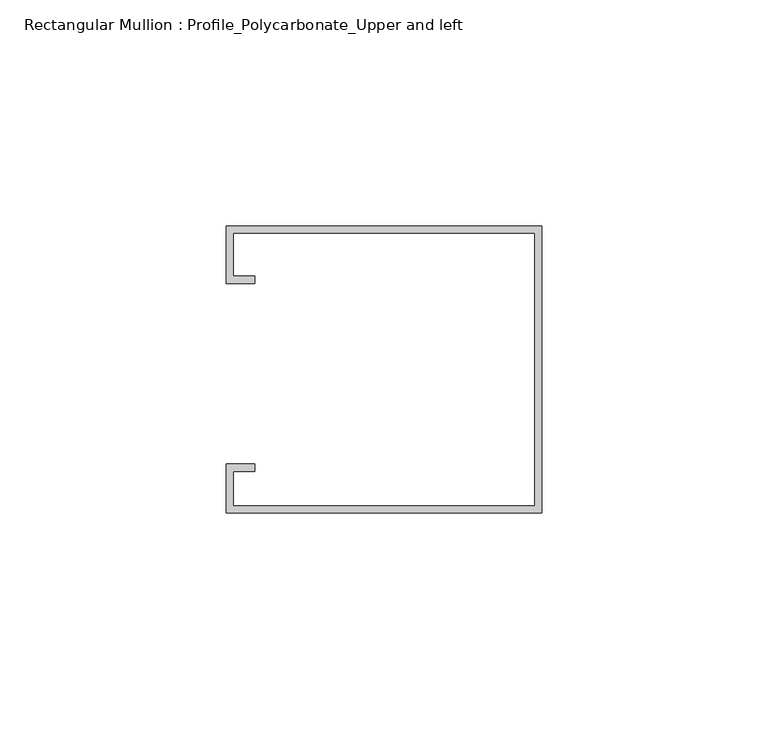
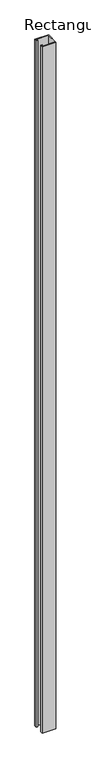
"""IFC4 building model written with IfcOpenShell, lengths in millimetres: member geometry, Rectangular Mullion : Profile_Polycarbonate_Upper and left."""

import ifcopenshell
import ifcopenshell.guid

model = None  # the IFC model being written
_history = None  # IfcOwnerHistory: only IFC2X3 demands one
_inside = {}  # id of a spatial element -> (the spatial element, [elements in it])
_under = {}  # id of a project, library or spatial element -> (it, [spatial elements below it])
_declared = {}  # id of a project -> (the project, [libraries it declares])
_typed = {}  # id of a type object -> (the type object, [elements of that type])
_made_of = {}  # id of a material, layer set ... -> (it, [elements and type objects made of it])


def new_model(schema):
    """Start an empty IFC model of exactly this schema.

    Asked for "IFC4X3", IfcOpenShell would pick the latest addendum, in which some entities
    have other attributes; the version numbers below select the first issue.
    IFC2X3 requires an IfcOwnerHistory on every rooted entity: one is made here for all.
    """
    global model, _history
    if schema == "IFC4X3":
        model = ifcopenshell.file(schema_version=(4, 3, 0, 0))
    else:
        model = ifcopenshell.file(schema=schema)
    _inside.clear()
    _under.clear()
    _declared.clear()
    _typed.clear()
    _made_of.clear()
    _history = None
    if model.schema == "IFC2X3":
        org = make("IfcOrganization", Name="unknown")
        user = make(
            "IfcPersonAndOrganization",
            ThePerson=make("IfcPerson", FamilyName="unknown"),
            TheOrganization=org,
        )
        app = make(
            "IfcApplication",
            ApplicationDeveloper=org,
            Version="unknown",
            ApplicationFullName="unknown",
            ApplicationIdentifier="unknown",
        )
        _history = make(
            "IfcOwnerHistory",
            OwningUser=user,
            OwningApplication=app,
            ChangeAction="ADDED",
            CreationDate=0,
        )
    return model


def make(cls, **values):
    """One entity of the class cls with the attributes given. An attribute that is None is left unset."""
    return model.create_entity(
        cls, **{name: value for name, value in values.items() if value is not None}
    )


def rooted(cls, **values):
    """An entity with a GlobalId (a new one), such as an element, a storey or a relation."""
    return make(cls, GlobalId=ifcopenshell.guid.new(), OwnerHistory=_history, **values)


def si_unit(unit_type, name, prefix=None):
    """IfcSIUnit, for example si_unit("LENGTHUNIT", "METRE", prefix="MILLI")."""
    return make("IfcSIUnit", UnitType=unit_type, Prefix=prefix, Name=name)


def assignment(units):
    """IfcUnitAssignment: the units of a project."""
    return None if units is None else make("IfcUnitAssignment", Units=units)


def point(xyz):
    """IfcCartesianPoint."""
    return None if xyz is None else make("IfcCartesianPoint", Coordinates=xyz)


def direction(xyz):
    """IfcDirection."""
    return None if xyz is None else make("IfcDirection", DirectionRatios=xyz)


def frame(location, z_axis=None, x_axis=None):
    """IfcAxis2Placement3D, a coordinate frame: its origin and axes. An axis left out is left unset."""
    return make(
        "IfcAxis2Placement3D",
        Location=point(location),
        Axis=direction(z_axis),
        RefDirection=direction(x_axis),
    )


def origin():
    """The frame at (0, 0, 0) with its axes left unset."""
    return frame((0.0, 0.0, 0.0))


def place(relative_to, where):
    """IfcLocalPlacement: puts the frame where relative to a parent placement (None: the world)."""
    return make(
        "IfcLocalPlacement", PlacementRelTo=relative_to, RelativePlacement=where
    )


def context(
    kind, dimensions, precision=None, world=None, true_north=None, identifier=None
):
    """IfcGeometricRepresentationContext, for example the 3D "Model" context."""
    return make(
        "IfcGeometricRepresentationContext",
        ContextIdentifier=identifier,
        ContextType=kind,
        CoordinateSpaceDimension=dimensions,
        Precision=precision,
        WorldCoordinateSystem=world,
        TrueNorth=true_north,
    )


def project(units=None, contexts=None):
    """IfcProject with its units and contexts."""
    return rooted(
        "IfcProject",
        Name="project",
        RepresentationContexts=contexts,
        UnitsInContext=assignment(units),
    )


def spatial(cls, under=None, at=None, **own):
    """A site, building, storey or space (cls), placed at a placement, below another one or the project."""
    s = rooted(cls, ObjectPlacement=at, **own)
    if under is not None:
        _under.setdefault(under.id(), (under, []))[1].append(s)
    return s


def polyline(points):
    """IfcPolyline through the points."""
    return make("IfcPolyline", Points=[point(p) for p in points])


def outline(outer, holes=None, kind="AREA"):
    """IfcArbitraryClosedProfileDef: a profile drawn as a closed curve; with holes, ...WithVoids."""
    if holes is None:
        return make("IfcArbitraryClosedProfileDef", ProfileType=kind, OuterCurve=outer)
    return make(
        "IfcArbitraryProfileDefWithVoids",
        ProfileType=kind,
        OuterCurve=outer,
        InnerCurves=holes,
    )


def extrude(swept, where, along, depth):
    """IfcExtrudedAreaSolid: the profile swept, set in the frame where, extruded along a direction by depth."""
    return make(
        "IfcExtrudedAreaSolid",
        SweptArea=swept,
        Position=where,
        ExtrudedDirection=direction(along),
        Depth=depth,
    )


def shape(context_of_items, identifier, shape_type, items):
    """IfcShapeRepresentation: the items that make up one representation, for example the "Body"."""
    return make(
        "IfcShapeRepresentation",
        ContextOfItems=context_of_items,
        RepresentationIdentifier=identifier,
        RepresentationType=shape_type,
        Items=items,
    )


def source(mapping_origin, context_of_items, identifier, shape_type, items):
    """IfcRepresentationMap: a shape defined once, which mapped items show again and again."""
    return make(
        "IfcRepresentationMap",
        MappingOrigin=mapping_origin,
        MappedRepresentation=shape(context_of_items, identifier, shape_type, items),
    )


def transform(
    local_origin,
    x_axis=None,
    y_axis=None,
    z_axis=None,
    scale=None,
    scale2=None,
    scale3=None,
    uniform=True,
):
    """IfcCartesianTransformationOperator3D, or its non-uniform kind. x_axis, y_axis, z_axis: its Axis1, 2, 3."""
    if uniform:
        return make(
            "IfcCartesianTransformationOperator3D",
            Axis1=direction(x_axis),
            Axis2=direction(y_axis),
            LocalOrigin=point(local_origin),
            Scale=scale,
            Axis3=direction(z_axis),
        )
    return make(
        "IfcCartesianTransformationOperator3DnonUniform",
        Axis1=direction(x_axis),
        Axis2=direction(y_axis),
        LocalOrigin=point(local_origin),
        Scale=scale,
        Axis3=direction(z_axis),
        Scale2=scale2,
        Scale3=scale3,
    )


def mapped(mapping_source, mapping_target):
    """IfcMappedItem: shows the shape of a source again, moved by a transform."""
    return make(
        "IfcMappedItem", MappingSource=mapping_source, MappingTarget=mapping_target
    )


def made_of(thing, what):
    """Note that an element or type object is made of a material, layer set ...; save() writes the relation."""
    if what is not None:
        _made_of.setdefault(what.id(), (what, []))[1].append(thing)
    return thing


def element(
    cls,
    number,
    at=None,
    inside=None,
    cuts=None,
    type_object=None,
    material=None,
    context=None,
    identifier="Body",
    shape_type=None,
    held_by="IfcProductDefinitionShape",
    body=None,
    shapes=None,
    **own,
):
    """One element of the class cls, such as IfcWall. Its Tag is "e" and its number.

    at: its placement. inside: the storey or other place that contains it. cuts: it is an
    opening in that element (IfcRelVoidsElement). A single representation is given by context,
    identifier, shape_type and body (its items); several are given by shapes. held_by: the class
    of the entity that holds the representations. save() writes the other relations.
    """
    e = rooted(cls, Tag="e%d" % number, ObjectPlacement=at, **own)
    if body is not None:
        shapes = [shape(context, identifier, shape_type, body)]
    if shapes is not None:
        e.Representation = make(held_by, Representations=shapes)
    if inside is not None:
        _inside.setdefault(inside.id(), (inside, []))[1].append(e)
    if cuts is not None:
        rooted(
            "IfcRelVoidsElement", RelatingBuildingElement=cuts, RelatedOpeningElement=e
        )
    if type_object is not None:
        _typed.setdefault(type_object.id(), (type_object, []))[1].append(e)
    return made_of(e, material)


def aggregate(whole, parts):
    """IfcRelAggregates: a whole, such as a stair, and the parts it consists of."""
    return rooted("IfcRelAggregates", RelatingObject=whole, RelatedObjects=parts)


def save(model, path):
    """Write the relations noted so far, then the file.

    IfcRelAggregates (storeys below a building ...), IfcRelContainedInSpatialStructure (elements
    in a storey), IfcRelDefinesByType, IfcRelAssociatesMaterial and IfcRelDeclares: one each for
    every whole, place, type object, material and project.
    """
    for whole, parts in _under.values():
        aggregate(whole, parts)
    for where, things in _inside.values():
        rooted(
            "IfcRelContainedInSpatialStructure",
            RelatedElements=things,
            RelatingStructure=where,
        )
    for kind, things in _typed.values():
        rooted("IfcRelDefinesByType", RelatedObjects=things, RelatingType=kind)
    for what, things in _made_of.values():
        rooted("IfcRelAssociatesMaterial", RelatedObjects=things, RelatingMaterial=what)
    for by, libraries in _declared.values():
        rooted("IfcRelDeclares", RelatingContext=by, RelatedDefinitions=libraries)
    model.write(path)


def rectangular_mullion_profile_polycarbonate_upper_and_left_b803591d(model_context):
    return source(origin(), model_context, "Body", "SweptSolid", [
        extrude(outline(polyline([(0.0, 32.7), (0.0, -30.8), (-69.85, -30.8), (-69.85, -20.0), (-63.5, -20.0), (-63.5, -21.5875), (-68.2625, -21.5875), (-68.2625, -29.2125), (-1.5875, -29.2125), (-1.5875, 31.1125), (-68.2625, 31.1125), (-68.2625, 21.5875), (-63.5, 21.5875), (-63.5, 20.0), (-69.85, 20.0), (-69.85, 32.7), (0.0, 32.7)])), frame((0.0, 0.0, -3695.7), z_axis=(0.0, 0.0, 1.0), x_axis=(1.0, 0.0, 0.0)), (0.0, 0.0, 1.0), 3695.7),
    ])


if __name__ == "__main__":
    model = new_model("IFC4")
    model_context = context("Model", 3, world=origin())
    ifc_project = project(units=[si_unit("LENGTHUNIT", "METRE", prefix="MILLI")], contexts=[model_context])
    site = spatial("IfcSite", under=ifc_project)
    building = spatial("IfcBuilding", under=site)
    placement = place(None, origin())
    rectangular_mullion_profile_polycarbonate_upper_and_left_shape = rectangular_mullion_profile_polycarbonate_upper_and_left_b803591d(model_context)
    element("IfcMember", 1, ObjectType="Rectangular Mullion : Profile_Polycarbonate_Upper and left", at=placement, inside=building, context=model_context, shape_type="MappedRepresentation", body=[
        mapped(rectangular_mullion_profile_polycarbonate_upper_and_left_shape, transform((0.0, 0.0, 0.0), x_axis=(1.0, 0.0, 0.0), y_axis=(0.0, 1.0, 0.0), z_axis=(0.0, 0.0, 1.0))),
    ])
    save(model, "model.ifc")

# Revit data of these elements
# Type "Rectangular Mullion : Profile_Polycarbonate_Upper and left"
#   built-in parameter 1007322 = 0.208333 (stored number, unit not read)
#   built-in parameter 1007321 = 0.00520833 (stored number, unit not read)
#   built-in parameter 1007320 = 0 (stored number, unit not read)
